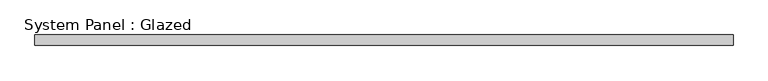
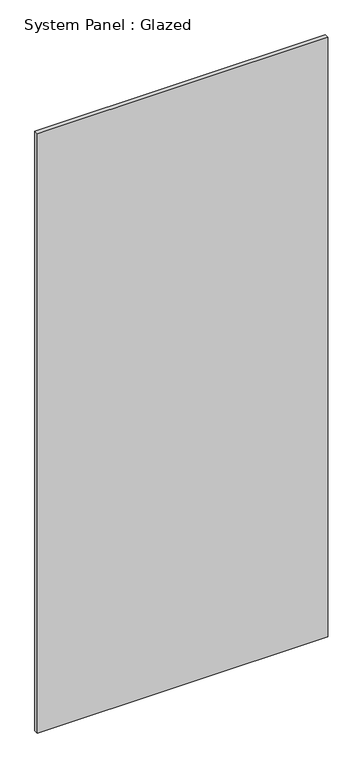
"""IFC4 building model written with IfcOpenShell, lengths in millimetres: plate geometry, System Panel : Glazed."""

from ifc_helpers import new_model, si_unit, origin, origin_with_axes, place, context, project, spatial, polyline, outline, extrude, source, transform, mapped, element, save


def system_panel_glazed_2e91cb65(model_context):
    return source(origin(), model_context, "Body", "SweptSolid", [
        extrude(outline(polyline([(838.2000002, -44.45), (-838.2000002, -44.45), (-838.2000002, -19.05), (838.2000002, -19.05), (838.2000002, -44.45)])), origin_with_axes(), (0.0, 0.0, 1.0), 3657.6),
    ])


if __name__ == "__main__":
    model = new_model("IFC4")
    model_context = context("Model", 3, world=origin())
    ifc_project = project(units=[si_unit("LENGTHUNIT", "METRE", prefix="MILLI")], contexts=[model_context])
    site = spatial("IfcSite", under=ifc_project)
    building = spatial("IfcBuilding", under=site)
    placement = place(None, origin())
    system_panel_glazed_shape = system_panel_glazed_2e91cb65(model_context)
    element("IfcPlate", 1, ObjectType="System Panel : Glazed", at=placement, inside=building, context=model_context, shape_type="MappedRepresentation", body=[
        mapped(system_panel_glazed_shape, transform((0.0, 0.0, 0.0), x_axis=(1.0, 0.0, 0.0), y_axis=(0.0, 1.0, 0.0), z_axis=(0.0, 0.0, 1.0))),
    ])
    save(model, "model.ifc")

# Revit data of these elements
# Type "System Panel : Glazed"
#   Construction Type Id = "GSP4R"
#   Analytic Construction = "1/8 in Pilkington single glazing"
#   Visual Light Transmittance = 0.9
#   Solar Heat Gain Coefficient = 0.86
#   Heat Transfer Coefficient (U) = 1.18115 BTU/(h·ft²·°F)
#   Define Thermal Properties by = 1
# Element 1 (IfcPlate, "System Panel : Glazed")
#   Materials on its faces: "Glass"
# Materials
#   "Glass": class "Glass", colour RGB 0 128 192, transparency 0.75, Description = "Soda Lime Glass", Cost = 0
